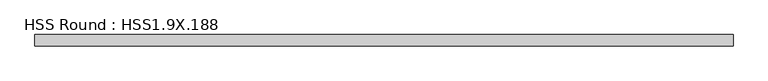
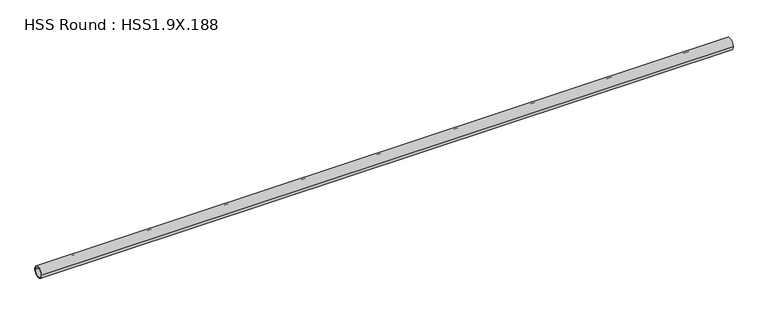
"""IFC4 building model written with IfcOpenShell, lengths in millimetres: member geometry, HSS Round : HSS1.9X.188."""

import ifcopenshell
import ifcopenshell.guid

model = None  # the IFC model being written
_history = None  # IfcOwnerHistory: only IFC2X3 demands one
_inside = {}  # id of a spatial element -> (the spatial element, [elements in it])
_under = {}  # id of a project, library or spatial element -> (it, [spatial elements below it])
_declared = {}  # id of a project -> (the project, [libraries it declares])
_typed = {}  # id of a type object -> (the type object, [elements of that type])
_made_of = {}  # id of a material, layer set ... -> (it, [elements and type objects made of it])


def new_model(schema):
    """Start an empty IFC model of exactly this schema.

    Asked for "IFC4X3", IfcOpenShell would pick the latest addendum, in which some entities
    have other attributes; the version numbers below select the first issue.
    IFC2X3 requires an IfcOwnerHistory on every rooted entity: one is made here for all.
    """
    global model, _history
    if schema == "IFC4X3":
        model = ifcopenshell.file(schema_version=(4, 3, 0, 0))
    else:
        model = ifcopenshell.file(schema=schema)
    _inside.clear()
    _under.clear()
    _declared.clear()
    _typed.clear()
    _made_of.clear()
    _history = None
    if model.schema == "IFC2X3":
        org = make("IfcOrganization", Name="unknown")
        user = make(
            "IfcPersonAndOrganization",
            ThePerson=make("IfcPerson", FamilyName="unknown"),
            TheOrganization=org,
        )
        app = make(
            "IfcApplication",
            ApplicationDeveloper=org,
            Version="unknown",
            ApplicationFullName="unknown",
            ApplicationIdentifier="unknown",
        )
        _history = make(
            "IfcOwnerHistory",
            OwningUser=user,
            OwningApplication=app,
            ChangeAction="ADDED",
            CreationDate=0,
        )
    return model


def make(cls, **values):
    """One entity of the class cls with the attributes given. An attribute that is None is left unset."""
    return model.create_entity(
        cls, **{name: value for name, value in values.items() if value is not None}
    )


def rooted(cls, **values):
    """An entity with a GlobalId (a new one), such as an element, a storey or a relation."""
    return make(cls, GlobalId=ifcopenshell.guid.new(), OwnerHistory=_history, **values)


def si_unit(unit_type, name, prefix=None):
    """IfcSIUnit, for example si_unit("LENGTHUNIT", "METRE", prefix="MILLI")."""
    return make("IfcSIUnit", UnitType=unit_type, Prefix=prefix, Name=name)


def assignment(units):
    """IfcUnitAssignment: the units of a project."""
    return None if units is None else make("IfcUnitAssignment", Units=units)


def point(xyz):
    """IfcCartesianPoint."""
    return None if xyz is None else make("IfcCartesianPoint", Coordinates=xyz)


def direction(xyz):
    """IfcDirection."""
    return None if xyz is None else make("IfcDirection", DirectionRatios=xyz)


def frame(location, z_axis=None, x_axis=None):
    """IfcAxis2Placement3D, a coordinate frame: its origin and axes. An axis left out is left unset."""
    return make(
        "IfcAxis2Placement3D",
        Location=point(location),
        Axis=direction(z_axis),
        RefDirection=direction(x_axis),
    )


def frame_2d(location, x_axis=None):
    """IfcAxis2Placement2D, a coordinate frame in the plane: its origin and x axis."""
    return make(
        "IfcAxis2Placement2D", Location=point(location), RefDirection=direction(x_axis)
    )


def origin():
    """The frame at (0, 0, 0) with its axes left unset."""
    return frame((0.0, 0.0, 0.0))


def origin_2d():
    """The frame at (0, 0) in the plane with its x axis left unset."""
    return frame_2d((0.0, 0.0))


def place(relative_to, where):
    """IfcLocalPlacement: puts the frame where relative to a parent placement (None: the world)."""
    return make(
        "IfcLocalPlacement", PlacementRelTo=relative_to, RelativePlacement=where
    )


def context(
    kind, dimensions, precision=None, world=None, true_north=None, identifier=None
):
    """IfcGeometricRepresentationContext, for example the 3D "Model" context."""
    return make(
        "IfcGeometricRepresentationContext",
        ContextIdentifier=identifier,
        ContextType=kind,
        CoordinateSpaceDimension=dimensions,
        Precision=precision,
        WorldCoordinateSystem=world,
        TrueNorth=true_north,
    )


def project(units=None, contexts=None):
    """IfcProject with its units and contexts."""
    return rooted(
        "IfcProject",
        Name="project",
        RepresentationContexts=contexts,
        UnitsInContext=assignment(units),
    )


def spatial(cls, under=None, at=None, **own):
    """A site, building, storey or space (cls), placed at a placement, below another one or the project."""
    s = rooted(cls, ObjectPlacement=at, **own)
    if under is not None:
        _under.setdefault(under.id(), (under, []))[1].append(s)
    return s


def circle_curve(where, radius):
    """IfcCircle in the frame where."""
    return make("IfcCircle", Position=where, Radius=radius)


def trimmed(basis, trim1, trim2, sense, master):
    """IfcTrimmedCurve: the piece of a basis curve between two trims."""
    return make(
        "IfcTrimmedCurve",
        BasisCurve=basis,
        Trim1=trim1,
        Trim2=trim2,
        SenseAgreement=sense,
        MasterRepresentation=master,
    )


def segment(curve, same_sense, transition):
    """IfcCompositeCurveSegment."""
    return make(
        "IfcCompositeCurveSegment",
        Transition=transition,
        SameSense=same_sense,
        ParentCurve=curve,
    )


def composite_curve(segments, self_intersect=None):
    """IfcCompositeCurve: segments joined end to end."""
    return make("IfcCompositeCurve", Segments=segments, SelfIntersect=self_intersect)


def outline(outer, holes=None, kind="AREA"):
    """IfcArbitraryClosedProfileDef: a profile drawn as a closed curve; with holes, ...WithVoids."""
    if holes is None:
        return make("IfcArbitraryClosedProfileDef", ProfileType=kind, OuterCurve=outer)
    return make(
        "IfcArbitraryProfileDefWithVoids",
        ProfileType=kind,
        OuterCurve=outer,
        InnerCurves=holes,
    )


def extrude(swept, where, along, depth):
    """IfcExtrudedAreaSolid: the profile swept, set in the frame where, extruded along a direction by depth."""
    return make(
        "IfcExtrudedAreaSolid",
        SweptArea=swept,
        Position=where,
        ExtrudedDirection=direction(along),
        Depth=depth,
    )


def shape(context_of_items, identifier, shape_type, items):
    """IfcShapeRepresentation: the items that make up one representation, for example the "Body"."""
    return make(
        "IfcShapeRepresentation",
        ContextOfItems=context_of_items,
        RepresentationIdentifier=identifier,
        RepresentationType=shape_type,
        Items=items,
    )


def source(mapping_origin, context_of_items, identifier, shape_type, items):
    """IfcRepresentationMap: a shape defined once, which mapped items show again and again."""
    return make(
        "IfcRepresentationMap",
        MappingOrigin=mapping_origin,
        MappedRepresentation=shape(context_of_items, identifier, shape_type, items),
    )


def transform(
    local_origin,
    x_axis=None,
    y_axis=None,
    z_axis=None,
    scale=None,
    scale2=None,
    scale3=None,
    uniform=True,
):
    """IfcCartesianTransformationOperator3D, or its non-uniform kind. x_axis, y_axis, z_axis: its Axis1, 2, 3."""
    if uniform:
        return make(
            "IfcCartesianTransformationOperator3D",
            Axis1=direction(x_axis),
            Axis2=direction(y_axis),
            LocalOrigin=point(local_origin),
            Scale=scale,
            Axis3=direction(z_axis),
        )
    return make(
        "IfcCartesianTransformationOperator3DnonUniform",
        Axis1=direction(x_axis),
        Axis2=direction(y_axis),
        LocalOrigin=point(local_origin),
        Scale=scale,
        Axis3=direction(z_axis),
        Scale2=scale2,
        Scale3=scale3,
    )


def mapped(mapping_source, mapping_target):
    """IfcMappedItem: shows the shape of a source again, moved by a transform."""
    return make(
        "IfcMappedItem", MappingSource=mapping_source, MappingTarget=mapping_target
    )


def made_of(thing, what):
    """Note that an element or type object is made of a material, layer set ...; save() writes the relation."""
    if what is not None:
        _made_of.setdefault(what.id(), (what, []))[1].append(thing)
    return thing


def element(
    cls,
    number,
    at=None,
    inside=None,
    cuts=None,
    type_object=None,
    material=None,
    context=None,
    identifier="Body",
    shape_type=None,
    held_by="IfcProductDefinitionShape",
    body=None,
    shapes=None,
    **own,
):
    """One element of the class cls, such as IfcWall. Its Tag is "e" and its number.

    at: its placement. inside: the storey or other place that contains it. cuts: it is an
    opening in that element (IfcRelVoidsElement). A single representation is given by context,
    identifier, shape_type and body (its items); several are given by shapes. held_by: the class
    of the entity that holds the representations. save() writes the other relations.
    """
    e = rooted(cls, Tag="e%d" % number, ObjectPlacement=at, **own)
    if body is not None:
        shapes = [shape(context, identifier, shape_type, body)]
    if shapes is not None:
        e.Representation = make(held_by, Representations=shapes)
    if inside is not None:
        _inside.setdefault(inside.id(), (inside, []))[1].append(e)
    if cuts is not None:
        rooted(
            "IfcRelVoidsElement", RelatingBuildingElement=cuts, RelatedOpeningElement=e
        )
    if type_object is not None:
        _typed.setdefault(type_object.id(), (type_object, []))[1].append(e)
    return made_of(e, material)


def aggregate(whole, parts):
    """IfcRelAggregates: a whole, such as a stair, and the parts it consists of."""
    return rooted("IfcRelAggregates", RelatingObject=whole, RelatedObjects=parts)


def save(model, path):
    """Write the relations noted so far, then the file.

    IfcRelAggregates (storeys below a building ...), IfcRelContainedInSpatialStructure (elements
    in a storey), IfcRelDefinesByType, IfcRelAssociatesMaterial and IfcRelDeclares: one each for
    every whole, place, type object, material and project.
    """
    for whole, parts in _under.values():
        aggregate(whole, parts)
    for where, things in _inside.values():
        rooted(
            "IfcRelContainedInSpatialStructure",
            RelatedElements=things,
            RelatingStructure=where,
        )
    for kind, things in _typed.values():
        rooted("IfcRelDefinesByType", RelatedObjects=things, RelatingType=kind)
    for what, things in _made_of.values():
        rooted("IfcRelAssociatesMaterial", RelatedObjects=things, RelatingMaterial=what)
    for by, libraries in _declared.values():
        rooted("IfcRelDeclares", RelatingContext=by, RelatedDefinitions=libraries)
    model.write(path)


def hss_round_hss1_9x_188_459573ad(model_context):
    return source(origin(), model_context, "Body", "SweptSolid", [
        extrude(outline(composite_curve([segment(trimmed(circle_curve(origin_2d(), 24.13), [point((-24.13, 0.0))], [point((24.13, 0.0))], False, "CARTESIAN"), True, "CONTINUOUS"), segment(trimmed(circle_curve(origin_2d(), 24.13), [point((24.13, 0.0))], [point((-24.13, 0.0))], False, "CARTESIAN"), True, "CONTINUOUS")], self_intersect=False), holes=[composite_curve([segment(trimmed(circle_curve(origin_2d(), 19.3548), [point((19.3548, 0.0))], [point((-19.3548, 0.0))], True, "CARTESIAN"), True, "CONTINUOUS"), segment(trimmed(circle_curve(origin_2d(), 19.3548), [point((-19.3548, 0.0))], [point((19.3548, 0.0))], True, "CARTESIAN"), True, "CONTINUOUS")], self_intersect=False)]), frame((-1502.7928259, 0.0, 0.0), z_axis=(1.0, 0.0, 0.0), x_axis=(0.0, 1.0, 0.0)), (0.0, 0.0, 1.0), 2931.7346976),
    ])


if __name__ == "__main__":
    model = new_model("IFC4")
    model_context = context("Model", 3, world=origin())
    ifc_project = project(units=[si_unit("LENGTHUNIT", "METRE", prefix="MILLI")], contexts=[model_context])
    site = spatial("IfcSite", under=ifc_project)
    building = spatial("IfcBuilding", under=site)
    placement = place(None, origin())
    hss_round_hss1_9x_188_shape = hss_round_hss1_9x_188_459573ad(model_context)
    element("IfcMember", 1, ObjectType="HSS Round : HSS1.9X.188", at=placement, inside=building, context=model_context, shape_type="MappedRepresentation", body=[
        mapped(hss_round_hss1_9x_188_shape, transform((0.0, 0.0, 0.0), x_axis=(1.0, 0.0, 0.0), y_axis=(0.0, 1.0, 0.0), z_axis=(0.0, 0.0, 1.0))),
    ])
    save(model, "model.ifc")

# Revit data of these elements
# Type "HSS Round : HSS1.9X.188"
#   Section Name Key = "HSSRound 1.900x0.188"
#   Assembly Code = "B10"
#   Wall Nominal Thickness = 0.188"
#   Wall Design Thickness = 0.174"
#   Torsional Moment of Inertia = 0.71 in⁴
#   Torsional Modulus = 0.747 in³
#   Section Area = 0.943 in²
#   Plastic Modulus weak axis = 0.52 in³
#   Plastic Modulus strong axis = 0.52 in³
#   Nominal Weight = 3.44 lbf/ft
#   Moment of Inertia weak axis = 0.355 in⁴
#   Moment of Inertia strong axis = 0.355 in⁴
#   Elastic Modulus weak axis = 0.374 in³
#   Elastic Modulus strong axis = 0.374 in³
#   Diameter = 1.900"
#   Centroid Vertical = 0.950"
#   Centroid Horizontal = 0.950"
#   Length [instance default] = 5' - 0"
#   Structural Material [instance default] = Steel ASTM A500, Grade B, Round
#   Warping Constant = (empty or 0)
#   Principal Axes Angle = 0
# Element 1 (IfcMember, "HSS Round : HSS1.9X.188")
#   Structural Material = Steel ASTM A992
#   Materials on its faces: "Steel ASTM A992"
# Materials
#   "Steel ASTM A500, Grade B, Round": class "Metal", colour RGB 199 199 199, transparency 0, Description = "Carbon steel", Cost = 0
#   "Steel ASTM A992": class "Metal", colour RGB 199 199 199, transparency 0, Description = "Structural steel 50ksi", Cost = 0
